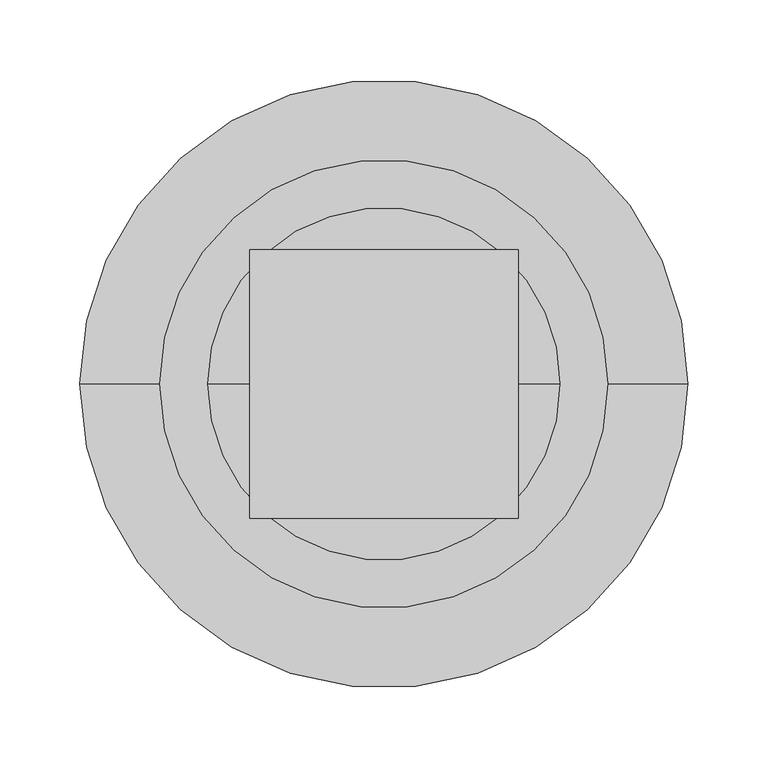
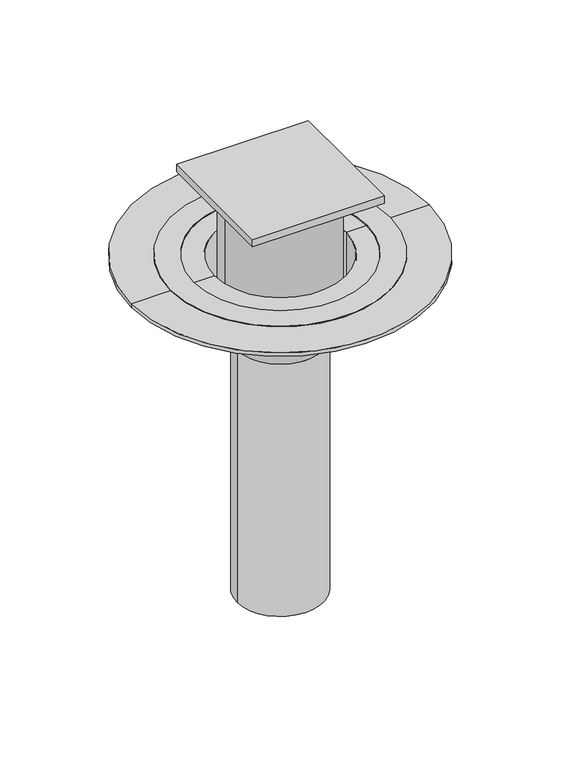
"""IFC4 building model written with IfcOpenShell, lengths in millimetres: proxy geometry, TN_Надставной элемент водоприемной воронки : Надставной элемент с обжимным металлическим фланцем, уплотнительным кольцом и трапом для эксплуатируемой кровли."""

import ifcopenshell
import ifcopenshell.guid

model = None  # the IFC model being written
_history = None  # IfcOwnerHistory: only IFC2X3 demands one
_inside = {}  # id of a spatial element -> (the spatial element, [elements in it])
_under = {}  # id of a project, library or spatial element -> (it, [spatial elements below it])
_declared = {}  # id of a project -> (the project, [libraries it declares])
_typed = {}  # id of a type object -> (the type object, [elements of that type])
_made_of = {}  # id of a material, layer set ... -> (it, [elements and type objects made of it])


def new_model(schema):
    """Start an empty IFC model of exactly this schema.

    Asked for "IFC4X3", IfcOpenShell would pick the latest addendum, in which some entities
    have other attributes; the version numbers below select the first issue.
    IFC2X3 requires an IfcOwnerHistory on every rooted entity: one is made here for all.
    """
    global model, _history
    if schema == "IFC4X3":
        model = ifcopenshell.file(schema_version=(4, 3, 0, 0))
    else:
        model = ifcopenshell.file(schema=schema)
    _inside.clear()
    _under.clear()
    _declared.clear()
    _typed.clear()
    _made_of.clear()
    _history = None
    if model.schema == "IFC2X3":
        org = make("IfcOrganization", Name="unknown")
        user = make(
            "IfcPersonAndOrganization",
            ThePerson=make("IfcPerson", FamilyName="unknown"),
            TheOrganization=org,
        )
        app = make(
            "IfcApplication",
            ApplicationDeveloper=org,
            Version="unknown",
            ApplicationFullName="unknown",
            ApplicationIdentifier="unknown",
        )
        _history = make(
            "IfcOwnerHistory",
            OwningUser=user,
            OwningApplication=app,
            ChangeAction="ADDED",
            CreationDate=0,
        )
    return model


def make(cls, **values):
    """One entity of the class cls with the attributes given. An attribute that is None is left unset."""
    return model.create_entity(
        cls, **{name: value for name, value in values.items() if value is not None}
    )


def rooted(cls, **values):
    """An entity with a GlobalId (a new one), such as an element, a storey or a relation."""
    return make(cls, GlobalId=ifcopenshell.guid.new(), OwnerHistory=_history, **values)


def si_unit(unit_type, name, prefix=None):
    """IfcSIUnit, for example si_unit("LENGTHUNIT", "METRE", prefix="MILLI")."""
    return make("IfcSIUnit", UnitType=unit_type, Prefix=prefix, Name=name)


def assignment(units):
    """IfcUnitAssignment: the units of a project."""
    return None if units is None else make("IfcUnitAssignment", Units=units)


def point(xyz):
    """IfcCartesianPoint."""
    return None if xyz is None else make("IfcCartesianPoint", Coordinates=xyz)


def direction(xyz):
    """IfcDirection."""
    return None if xyz is None else make("IfcDirection", DirectionRatios=xyz)


def frame(location, z_axis=None, x_axis=None):
    """IfcAxis2Placement3D, a coordinate frame: its origin and axes. An axis left out is left unset."""
    return make(
        "IfcAxis2Placement3D",
        Location=point(location),
        Axis=direction(z_axis),
        RefDirection=direction(x_axis),
    )


def frame_2d(location, x_axis=None):
    """IfcAxis2Placement2D, a coordinate frame in the plane: its origin and x axis."""
    return make(
        "IfcAxis2Placement2D", Location=point(location), RefDirection=direction(x_axis)
    )


def origin():
    """The frame at (0, 0, 0) with its axes left unset."""
    return frame((0.0, 0.0, 0.0))


def origin_with_axes():
    """The frame at (0, 0, 0) with the z axis (0, 0, 1) and the x axis (1, 0, 0) written out."""
    return frame((0.0, 0.0, 0.0), z_axis=(0.0, 0.0, 1.0), x_axis=(1.0, 0.0, 0.0))


def origin_2d():
    """The frame at (0, 0) in the plane with its x axis left unset."""
    return frame_2d((0.0, 0.0))


def place(relative_to, where):
    """IfcLocalPlacement: puts the frame where relative to a parent placement (None: the world)."""
    return make(
        "IfcLocalPlacement", PlacementRelTo=relative_to, RelativePlacement=where
    )


def context(
    kind, dimensions, precision=None, world=None, true_north=None, identifier=None
):
    """IfcGeometricRepresentationContext, for example the 3D "Model" context."""
    return make(
        "IfcGeometricRepresentationContext",
        ContextIdentifier=identifier,
        ContextType=kind,
        CoordinateSpaceDimension=dimensions,
        Precision=precision,
        WorldCoordinateSystem=world,
        TrueNorth=true_north,
    )


def project(units=None, contexts=None):
    """IfcProject with its units and contexts."""
    return rooted(
        "IfcProject",
        Name="project",
        RepresentationContexts=contexts,
        UnitsInContext=assignment(units),
    )


def spatial(cls, under=None, at=None, **own):
    """A site, building, storey or space (cls), placed at a placement, below another one or the project."""
    s = rooted(cls, ObjectPlacement=at, **own)
    if under is not None:
        _under.setdefault(under.id(), (under, []))[1].append(s)
    return s


def polyline(points):
    """IfcPolyline through the points."""
    return make("IfcPolyline", Points=[point(p) for p in points])


def circle_curve(where, radius):
    """IfcCircle in the frame where."""
    return make("IfcCircle", Position=where, Radius=radius)


def trimmed(basis, trim1, trim2, sense, master):
    """IfcTrimmedCurve: the piece of a basis curve between two trims."""
    return make(
        "IfcTrimmedCurve",
        BasisCurve=basis,
        Trim1=trim1,
        Trim2=trim2,
        SenseAgreement=sense,
        MasterRepresentation=master,
    )


def segment(curve, same_sense, transition):
    """IfcCompositeCurveSegment."""
    return make(
        "IfcCompositeCurveSegment",
        Transition=transition,
        SameSense=same_sense,
        ParentCurve=curve,
    )


def composite_curve(segments, self_intersect=None):
    """IfcCompositeCurve: segments joined end to end."""
    return make("IfcCompositeCurve", Segments=segments, SelfIntersect=self_intersect)


def outline(outer, holes=None, kind="AREA"):
    """IfcArbitraryClosedProfileDef: a profile drawn as a closed curve; with holes, ...WithVoids."""
    if holes is None:
        return make("IfcArbitraryClosedProfileDef", ProfileType=kind, OuterCurve=outer)
    return make(
        "IfcArbitraryProfileDefWithVoids",
        ProfileType=kind,
        OuterCurve=outer,
        InnerCurves=holes,
    )


def extrude(swept, where, along, depth):
    """IfcExtrudedAreaSolid: the profile swept, set in the frame where, extruded along a direction by depth."""
    return make(
        "IfcExtrudedAreaSolid",
        SweptArea=swept,
        Position=where,
        ExtrudedDirection=direction(along),
        Depth=depth,
    )


def shape(context_of_items, identifier, shape_type, items):
    """IfcShapeRepresentation: the items that make up one representation, for example the "Body"."""
    return make(
        "IfcShapeRepresentation",
        ContextOfItems=context_of_items,
        RepresentationIdentifier=identifier,
        RepresentationType=shape_type,
        Items=items,
    )


def source(mapping_origin, context_of_items, identifier, shape_type, items):
    """IfcRepresentationMap: a shape defined once, which mapped items show again and again."""
    return make(
        "IfcRepresentationMap",
        MappingOrigin=mapping_origin,
        MappedRepresentation=shape(context_of_items, identifier, shape_type, items),
    )


def transform(
    local_origin,
    x_axis=None,
    y_axis=None,
    z_axis=None,
    scale=None,
    scale2=None,
    scale3=None,
    uniform=True,
):
    """IfcCartesianTransformationOperator3D, or its non-uniform kind. x_axis, y_axis, z_axis: its Axis1, 2, 3."""
    if uniform:
        return make(
            "IfcCartesianTransformationOperator3D",
            Axis1=direction(x_axis),
            Axis2=direction(y_axis),
            LocalOrigin=point(local_origin),
            Scale=scale,
            Axis3=direction(z_axis),
        )
    return make(
        "IfcCartesianTransformationOperator3DnonUniform",
        Axis1=direction(x_axis),
        Axis2=direction(y_axis),
        LocalOrigin=point(local_origin),
        Scale=scale,
        Axis3=direction(z_axis),
        Scale2=scale2,
        Scale3=scale3,
    )


def mapped(mapping_source, mapping_target):
    """IfcMappedItem: shows the shape of a source again, moved by a transform."""
    return make(
        "IfcMappedItem", MappingSource=mapping_source, MappingTarget=mapping_target
    )


def made_of(thing, what):
    """Note that an element or type object is made of a material, layer set ...; save() writes the relation."""
    if what is not None:
        _made_of.setdefault(what.id(), (what, []))[1].append(thing)
    return thing


def element(
    cls,
    number,
    at=None,
    inside=None,
    cuts=None,
    type_object=None,
    material=None,
    context=None,
    identifier="Body",
    shape_type=None,
    held_by="IfcProductDefinitionShape",
    body=None,
    shapes=None,
    **own,
):
    """One element of the class cls, such as IfcWall. Its Tag is "e" and its number.

    at: its placement. inside: the storey or other place that contains it. cuts: it is an
    opening in that element (IfcRelVoidsElement). A single representation is given by context,
    identifier, shape_type and body (its items); several are given by shapes. held_by: the class
    of the entity that holds the representations. save() writes the other relations.
    """
    e = rooted(cls, Tag="e%d" % number, ObjectPlacement=at, **own)
    if body is not None:
        shapes = [shape(context, identifier, shape_type, body)]
    if shapes is not None:
        e.Representation = make(held_by, Representations=shapes)
    if inside is not None:
        _inside.setdefault(inside.id(), (inside, []))[1].append(e)
    if cuts is not None:
        rooted(
            "IfcRelVoidsElement", RelatingBuildingElement=cuts, RelatedOpeningElement=e
        )
    if type_object is not None:
        _typed.setdefault(type_object.id(), (type_object, []))[1].append(e)
    return made_of(e, material)


def aggregate(whole, parts):
    """IfcRelAggregates: a whole, such as a stair, and the parts it consists of."""
    return rooted("IfcRelAggregates", RelatingObject=whole, RelatedObjects=parts)


def save(model, path):
    """Write the relations noted so far, then the file.

    IfcRelAggregates (storeys below a building ...), IfcRelContainedInSpatialStructure (elements
    in a storey), IfcRelDefinesByType, IfcRelAssociatesMaterial and IfcRelDeclares: one each for
    every whole, place, type object, material and project.
    """
    for whole, parts in _under.values():
        aggregate(whole, parts)
    for where, things in _inside.values():
        rooted(
            "IfcRelContainedInSpatialStructure",
            RelatedElements=things,
            RelatingStructure=where,
        )
    for kind, things in _typed.values():
        rooted("IfcRelDefinesByType", RelatedObjects=things, RelatingType=kind)
    for what, things in _made_of.values():
        rooted("IfcRelAssociatesMaterial", RelatedObjects=things, RelatingMaterial=what)
    for by, libraries in _declared.values():
        rooted("IfcRelDeclares", RelatingContext=by, RelatedDefinitions=libraries)
    model.write(path)


def plane_surface(at):
    """IfcPlane: the flat surface through the origin of the frame at, square to its z axis."""
    return make("IfcPlane", Position=at)


def cylinder_surface(at, radius):
    """IfcCylindricalSurface: all points at the distance radius from the z axis of the frame at."""
    return make("IfcCylindricalSurface", Position=at, Radius=radius)


def revolved_surface(curve, axis_point, axis_direction):
    """IfcSurfaceOfRevolution: the curve turned about the line through axis_point along axis_direction."""
    return make(
        "IfcSurfaceOfRevolution",
        SweptCurve=make("IfcArbitraryOpenProfileDef", ProfileType="CURVE", Curve=curve),
        AxisPosition=make("IfcAxis1Placement", Location=point(axis_point), Axis=direction(axis_direction)),
    )


def advanced_brep(points, edges, surfaces, faces):
    """IfcAdvancedBrep: a solid bounded by faces that lie on surfaces and meet in shared edges.

    An edge is (start, end): straight between two places in points (the first is 0);
    or (start, end, curve); or (start, end, curve, False) where it runs against its curve.
    A face is (place in surfaces, loops), or (place, loops, False) where it looks against
    its surface's normal. A loop lists edges by number (the first is 1), with a minus sign
    where the edge is run from its end to its start. The first loop is the outer one.
    """
    corners = [point(p) for p in points]
    vertices = [make("IfcVertexPoint", VertexGeometry=c) for c in corners]
    made = []
    for start, end, *more in edges:
        made.append(
            make(
                "IfcEdgeCurve",
                EdgeStart=vertices[start],
                EdgeEnd=vertices[end],
                EdgeGeometry=more[0] if more else make("IfcPolyline", Points=[corners[start], corners[end]]),
                SameSense=more[1] if len(more) > 1 else True,
            )
        )
    hull = []
    for where, loops, *sense in faces:
        bounds = []
        for j, loop in enumerate(loops):
            ring = [make("IfcOrientedEdge", EdgeElement=made[abs(k) - 1], Orientation=k > 0) for k in loop]
            bounds.append(
                make(
                    "IfcFaceOuterBound" if j == 0 else "IfcFaceBound",
                    Bound=make("IfcEdgeLoop", EdgeList=ring),
                    Orientation=True,
                )
            )
        hull.append(make("IfcAdvancedFace", Bounds=bounds, FaceSurface=surfaces[where], SameSense=sense[0] if sense else True))
    return make("IfcAdvancedBrep", Outer=make("IfcClosedShell", CfsFaces=hull))


def specialty_equipment_1411c5ad(model_context):
    return source(origin(), model_context, "Body", "SolidModel", [
        extrude(outline(composite_curve([segment(trimmed(circle_curve(origin_2d(), 70.0), [point((-70.0, 0.0))], [point((70.0, 0.0))], False, "CARTESIAN"), True, "CONTINUOUS"), segment(trimmed(circle_curve(origin_2d(), 70.0), [point((70.0, 0.0))], [point((-70.0, 0.0))], False, "CARTESIAN"), True, "CONTINUOUS")], self_intersect=False)), frame((0.0, 0.0, -66.9669914), z_axis=(0.0, 0.0, 1.0), x_axis=(1.0, 0.0, 0.0)), (0.0, 0.0, 1.0), 156.9669914),
        extrude(outline(polyline([(83.890873, 83.890873), (83.890873, -83.890873), (-83.890873, -83.890873), (-83.890873, 83.890873), (83.890873, 83.890873)])), frame((0.0, 0.0, 90.0), z_axis=(0.0, 0.0, 1.0), x_axis=(1.0, 0.0, 0.0)), (0.0, 0.0, 1.0), 10.0),
        extrude(outline(composite_curve([segment(trimmed(circle_curve(origin_2d(), 140.0), [point((-140.0, 0.0))], [point((140.0, 0.0))], False, "CARTESIAN"), True, "CONTINUOUS"), segment(trimmed(circle_curve(origin_2d(), 140.0), [point((140.0, 0.0))], [point((-140.0, 0.0))], False, "CARTESIAN"), True, "CONTINUOUS")], self_intersect=False), holes=[composite_curve([segment(trimmed(circle_curve(origin_2d(), 110.0556416), [point((-110.0556416, 0.0))], [point((110.0556416, 0.0))], True, "CARTESIAN"), True, "CONTINUOUS"), segment(trimmed(circle_curve(origin_2d(), 110.0556416), [point((110.0556416, 0.0))], [point((-110.0556416, 0.0))], True, "CARTESIAN"), True, "CONTINUOUS")], self_intersect=False)]), origin_with_axes(), (0.0, 0.0, 1.0), 1.0),
        advanced_brep(
        [(0.0, 0.0, -450.0), (-55.0, 0.0, -450.0), (55.0, 0.0, -450.0), (190.0, 0.0, 0.0), (-190.0, 0.0, 0.0), (-83.890873, 0.0, 0.0), (83.890873, 0.0, 0.0), (190.0, 0.0, -5.0), (-190.0, 0.0, -5.0), (93.890873, 0.0, -5.0), (-93.890873, 0.0, -5.0), (55.0, 0.0, -110.0), (-55.0, 0.0, -110.0), (-93.890873, 0.0, -71.109127), (93.890873, 0.0, -71.109127), (55.5025253, 0.0, -95.3553391), (-55.5025253, 0.0, -95.3553391), (0.0, 0.0, -95.3553391), (83.890873, 0.0, -66.9669914), (-83.890873, 0.0, -66.9669914)],
        [
            (0, 1),
            (1, 2, circle_curve(frame((0.0, 0.0, -450.0), z_axis=(0.0, 0.0, -1.0), x_axis=(-1.0, 0.0, 0.0)), 55.0)),
            (2, 0),
            (2, 1, circle_curve(frame((0.0, 0.0, -450.0), z_axis=(0.0, 0.0, -1.0), x_axis=(-1.0, 0.0, 0.0)), 55.0)),
            (3, 4, circle_curve(frame((0.0, 0.0, 0.0), z_axis=(0.0, 0.0, 1.0), x_axis=(-1.0, 0.0, 0.0)), 190.0)),
            (4, 5),
            (5, 6, circle_curve(frame((0.0, 0.0, 0.0), z_axis=(0.0, 0.0, -1.0), x_axis=(-1.0, 0.0, 0.0)), 83.890873)),
            (6, 3),
            (4, 3, circle_curve(frame((0.0, 0.0, 0.0), z_axis=(0.0, 0.0, 1.0), x_axis=(-1.0, 0.0, 0.0)), 190.0)),
            (6, 5, circle_curve(frame((0.0, 0.0, 0.0), z_axis=(0.0, 0.0, -1.0), x_axis=(-1.0, 0.0, 0.0)), 83.890873)),
            (7, 8, circle_curve(frame((0.0, 0.0, -5.0), z_axis=(0.0, 0.0, 1.0), x_axis=(-1.0, 0.0, 0.0)), 190.0)),
            (8, 4),
            (3, 7),
            (8, 7, circle_curve(frame((0.0, 0.0, -5.0), z_axis=(0.0, 0.0, 1.0), x_axis=(-1.0, 0.0, 0.0)), 190.0)),
            (9, 10, circle_curve(frame((0.0, 0.0, -5.0), z_axis=(0.0, 0.0, 1.0), x_axis=(-1.0, 0.0, 0.0)), 93.890873)),
            (10, 8),
            (7, 9),
            (10, 9, circle_curve(frame((0.0, 0.0, -5.0), z_axis=(0.0, 0.0, 1.0), x_axis=(-1.0, 0.0, 0.0)), 93.890873)),
            (11, 12, circle_curve(frame((0.0, 0.0, -110.0), z_axis=(0.0, 0.0, 1.0), x_axis=(-1.0, 0.0, 0.0)), 55.0)),
            (12, 13),
            (13, 14, circle_curve(frame((0.0, 0.0, -71.109127), z_axis=(0.0, 0.0, -1.0), x_axis=(-1.0, 0.0, 0.0)), 93.890873)),
            (14, 11),
            (12, 11, circle_curve(frame((0.0, 0.0, -110.0), z_axis=(0.0, 0.0, 1.0), x_axis=(-1.0, 0.0, 0.0)), 55.0)),
            (14, 13, circle_curve(frame((0.0, 0.0, -71.109127), z_axis=(0.0, 0.0, -1.0), x_axis=(-1.0, 0.0, 0.0)), 93.890873)),
            (1, 12),
            (11, 2),
            (13, 10),
            (9, 14),
            (15, 16, circle_curve(frame((0.0, 0.0, -95.3553391), z_axis=(0.0, 0.0, 1.0), x_axis=(-1.0, 0.0, 0.0)), 55.5025253)),
            (16, 17),
            (17, 15),
            (16, 15, circle_curve(frame((0.0, 0.0, -95.3553391), z_axis=(0.0, 0.0, 1.0), x_axis=(-1.0, 0.0, 0.0)), 55.5025253)),
            (18, 19, circle_curve(frame((0.0, 0.0, -66.9669914), z_axis=(0.0, 0.0, 1.0), x_axis=(-1.0, 0.0, 0.0)), 83.890873)),
            (19, 16),
            (15, 18),
            (19, 18, circle_curve(frame((0.0, 0.0, -66.9669914), z_axis=(0.0, 0.0, 1.0), x_axis=(-1.0, 0.0, 0.0)), 83.890873)),
            (5, 19),
            (18, 6),
        ],
        [
            plane_surface(frame((0.0, 0.0, -450.0), z_axis=(0.0, 0.0, -1.0), x_axis=(-1.0, 0.0, 0.0))),
            plane_surface(frame((0.0, 0.0, 0.0), z_axis=(0.0, 0.0, 1.0), x_axis=(-1.0, 0.0, 0.0))),
            cylinder_surface(frame((0.0, 0.0, 0.0), z_axis=(0.0, 0.0, -1.0), x_axis=(-1.0, 0.0, 0.0)), 190.0),
            plane_surface(frame((0.0, 0.0, -5.0), z_axis=(0.0, 0.0, -1.0), x_axis=(-1.0, 0.0, 0.0))),
            revolved_surface(polyline([(-93.890873, 0.0, -71.109127), (-55.0, 0.0, -110.0)]), (0.0, 0.0, 0.0), (0.0, 0.0, -1.0)),
            cylinder_surface(frame((0.0, 0.0, 0.0), z_axis=(0.0, 0.0, -1.0), x_axis=(-1.0, 0.0, 0.0)), 55.0),
            cylinder_surface(frame((0.0, 0.0, 0.0), z_axis=(0.0, 0.0, -1.0), x_axis=(-1.0, 0.0, 0.0)), 93.890873),
            plane_surface(frame((0.0, 0.0, -95.3553391), z_axis=(0.0, 0.0, 1.0), x_axis=(-1.0, 0.0, 0.0))),
            revolved_surface(polyline([(-55.5025253, 0.0, -95.3553391), (-83.890873, 0.0, -66.9669914)]), (0.0, 0.0, 0.0), (0.0, 0.0, -1.0)),
            revolved_surface(polyline([(-83.890873, 0.0, -66.9669914), (-83.890873, 0.0, 0.0)]), (0.0, 0.0, 0.0), (0.0, 0.0, -1.0)),
        ],
        [
            (0, [[1, 2, 3]]),
            (0, [[-3, 4, -1]]),
            (1, [[5, 6, 7, 8]]),
            (1, [[9, -8, 10, -6]]),
            (2, [[11, 12, -5, 13]]),
            (2, [[14, -13, -9, -12]]),
            (3, [[15, 16, -11, 17]]),
            (3, [[18, -17, -14, -16]]),
            (4, [[19, 20, 21, 22]]),
            (4, [[23, -22, 24, -20]]),
            (5, [[-2, 25, -19, 26]]),
            (5, [[-4, -26, -23, -25]]),
            (6, [[-21, 27, -15, 28]]),
            (6, [[-24, -28, -18, -27]]),
            (7, [[29, 30, 31]]),
            (7, [[32, -31, -30]]),
            (8, [[33, 34, -29, 35]]),
            (8, [[36, -35, -32, -34]]),
            (9, [[-7, 37, -33, 38]]),
            (9, [[-10, -38, -36, -37]]),
        ],
    ),
    ])


if __name__ == "__main__":
    model = new_model("IFC4")
    model_context = context("Model", 3, world=origin())
    ifc_project = project(units=[si_unit("LENGTHUNIT", "METRE", prefix="MILLI")], contexts=[model_context])
    site = spatial("IfcSite", under=ifc_project)
    building = spatial("IfcBuilding", under=site)
    placement = place(None, origin())
    specialty_equipment_shape = specialty_equipment_1411c5ad(model_context)
    element("IfcBuildingElementProxy", 1, Name="TN_Надставной элемент водоприемной воронки : Надставной элемент с обжимным металлическим фланцем, уплотнительным кольцом и трапом для эксплуатируемой кровли", ObjectType="TN_Надставной элемент водоприемной воронки : Надставной элемент с обжимным металлическим фланцем, уплотнительным кольцом и трапом для эксплуатируемой кровли", at=placement, inside=building, context=model_context, shape_type="MappedRepresentation", body=[
        mapped(specialty_equipment_shape, transform((0.0, 0.0, 0.0), x_axis=(1.0, 0.0, 0.0), y_axis=(0.0, 1.0, 0.0), z_axis=(0.0, 0.0, 1.0))),
    ])
    save(model, "model.ifc")

# Revit data of these elements
# Type "TN_Надставной элемент водоприемной воронки : Надставной элемент с обжимным металлическим фланцем, уплотнительным кольцом и трапом для эксплуатируемой кровли"
#   ADSK_Группирование = "Комплектующие и воронки"
#   Description = "Надставной элемент с обжимным металлическим фланцем и уплотнительным кольцом применяется для создания двух уровневых кровельных воронок. Манжета предотвращает проникновение ливневых стоков в слой теплоизоляции по месту соединения надставного элемента с воронкой. Может быть также использован как самостоятельное изделие подобно воронке с обжимным металлическим фланцем. Также надставной элемент комплектуется уплотнительным кольцом, комплектом гаек и барашков."
#   Manufacturer = "ТехноНИКОЛЬ"
#   URL = "https://shop.tn.ru/nadstavnoj-jelement-s-obzhimnym-metallicheskim-flancem-i-uplotnitelnym-kolcom"
#   ADSK_Примечание = ""
#   ADSK_Обозначение = "ТехноНИКОЛЬ"
#   ADSK_Наименование = "Надставной элемент с обжимным металлическим  фланцем, уплотнительным кольцом и трапом для эксплуатируемой кровли"
#   ADSK_Марка = ""
#   ADSK_Код изделия = "661133"
#   ADSK_Завод-изготовитель = "ТехноНИКОЛЬ"
#   ADSK_Единица измерения = "шт."
#   ADSK_Группирование = "Комплектующие и воронки"
#   ADSK_URL страницы изделия = "https://shop.tn.ru/nadstavnoj-jelement-s-obzhimnym-metallicheskim-flancem-i-uplotnitelnym-kolcom"
#   ADSK_URL документации изделия = "https://shop.tn.ru/media/other_documents/_661129_661126_661128_661127_661133.pdf"
#   Тип надставного элемента = 2
#   Радиус = 55 mm
#   Длина расчетная [instance default] = 450 mm
#   Длина отвода [instance default] = 450 mm
#   Высота трапа расчетная [instance default] = 50 mm
#   Высота трапа [instance default] = 50 mm
#   ADSK_Количество = 1
#   Видимость_Листоуловитель [instance default] = no
#   Видимость трапа [instance default] = yes
#   Видимость листоуловителя [instance default] = no
#   Материал_Фланец = TN_ПВХ_Серый
#   Материал_Корпус = TN_ПВХ_Черный
#   Default Elevation = 0
# Element 1 (IfcBuildingElementProxy, "TN_Надставной элемент водоприемной воронки : Надставной элемент с обжимным металлическим фланцем, уплотнительным кольцом и трапом для эксплуатируемой кровли")
#   Высота трапа расчетная = 100 mm
#   Высота трапа = 100 mm
#   Видимость_Листоуловитель = yes
#   Materials on its faces: "TN_ПВХ_Черный", "TN_ПВХ_Серый"
# Materials
#   "TN_ПВХ_Серый": class "Типовые", colour RGB 192 192 192, transparency 0, Cost = 0
#   "TN_ПВХ_Черный": class "Типовые", colour RGB 48 48 48, transparency 0, Cost = 0
